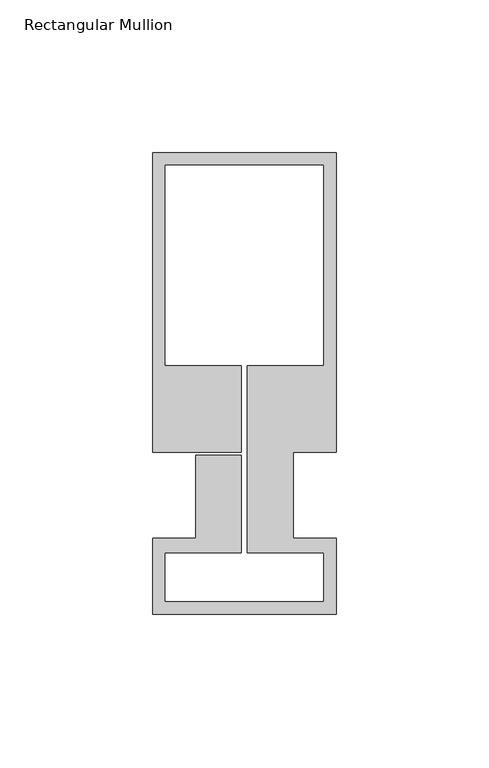
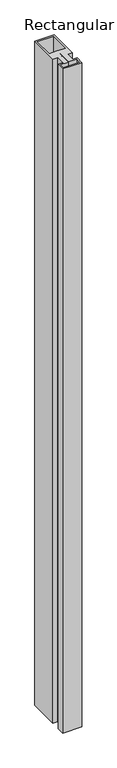
"""IFC4 building model written with IfcOpenShell, lengths in millimetres: member geometry, Rectangular Mullion : Schueco_FWS-60-HI_Mull_CovCap-20mm_Mull-85mm."""

import ifcopenshell
import ifcopenshell.guid

model = None  # the IFC model being written
_history = None  # IfcOwnerHistory: only IFC2X3 demands one
_inside = {}  # id of a spatial element -> (the spatial element, [elements in it])
_under = {}  # id of a project, library or spatial element -> (it, [spatial elements below it])
_declared = {}  # id of a project -> (the project, [libraries it declares])
_typed = {}  # id of a type object -> (the type object, [elements of that type])
_made_of = {}  # id of a material, layer set ... -> (it, [elements and type objects made of it])


def new_model(schema):
    """Start an empty IFC model of exactly this schema.

    Asked for "IFC4X3", IfcOpenShell would pick the latest addendum, in which some entities
    have other attributes; the version numbers below select the first issue.
    IFC2X3 requires an IfcOwnerHistory on every rooted entity: one is made here for all.
    """
    global model, _history
    if schema == "IFC4X3":
        model = ifcopenshell.file(schema_version=(4, 3, 0, 0))
    else:
        model = ifcopenshell.file(schema=schema)
    _inside.clear()
    _under.clear()
    _declared.clear()
    _typed.clear()
    _made_of.clear()
    _history = None
    if model.schema == "IFC2X3":
        org = make("IfcOrganization", Name="unknown")
        user = make(
            "IfcPersonAndOrganization",
            ThePerson=make("IfcPerson", FamilyName="unknown"),
            TheOrganization=org,
        )
        app = make(
            "IfcApplication",
            ApplicationDeveloper=org,
            Version="unknown",
            ApplicationFullName="unknown",
            ApplicationIdentifier="unknown",
        )
        _history = make(
            "IfcOwnerHistory",
            OwningUser=user,
            OwningApplication=app,
            ChangeAction="ADDED",
            CreationDate=0,
        )
    return model


def make(cls, **values):
    """One entity of the class cls with the attributes given. An attribute that is None is left unset."""
    return model.create_entity(
        cls, **{name: value for name, value in values.items() if value is not None}
    )


def rooted(cls, **values):
    """An entity with a GlobalId (a new one), such as an element, a storey or a relation."""
    return make(cls, GlobalId=ifcopenshell.guid.new(), OwnerHistory=_history, **values)


def si_unit(unit_type, name, prefix=None):
    """IfcSIUnit, for example si_unit("LENGTHUNIT", "METRE", prefix="MILLI")."""
    return make("IfcSIUnit", UnitType=unit_type, Prefix=prefix, Name=name)


def assignment(units):
    """IfcUnitAssignment: the units of a project."""
    return None if units is None else make("IfcUnitAssignment", Units=units)


def point(xyz):
    """IfcCartesianPoint."""
    return None if xyz is None else make("IfcCartesianPoint", Coordinates=xyz)


def direction(xyz):
    """IfcDirection."""
    return None if xyz is None else make("IfcDirection", DirectionRatios=xyz)


def frame(location, z_axis=None, x_axis=None):
    """IfcAxis2Placement3D, a coordinate frame: its origin and axes. An axis left out is left unset."""
    return make(
        "IfcAxis2Placement3D",
        Location=point(location),
        Axis=direction(z_axis),
        RefDirection=direction(x_axis),
    )


def origin():
    """The frame at (0, 0, 0) with its axes left unset."""
    return frame((0.0, 0.0, 0.0))


def place(relative_to, where):
    """IfcLocalPlacement: puts the frame where relative to a parent placement (None: the world)."""
    return make(
        "IfcLocalPlacement", PlacementRelTo=relative_to, RelativePlacement=where
    )


def context(
    kind, dimensions, precision=None, world=None, true_north=None, identifier=None
):
    """IfcGeometricRepresentationContext, for example the 3D "Model" context."""
    return make(
        "IfcGeometricRepresentationContext",
        ContextIdentifier=identifier,
        ContextType=kind,
        CoordinateSpaceDimension=dimensions,
        Precision=precision,
        WorldCoordinateSystem=world,
        TrueNorth=true_north,
    )


def project(units=None, contexts=None):
    """IfcProject with its units and contexts."""
    return rooted(
        "IfcProject",
        Name="project",
        RepresentationContexts=contexts,
        UnitsInContext=assignment(units),
    )


def spatial(cls, under=None, at=None, **own):
    """A site, building, storey or space (cls), placed at a placement, below another one or the project."""
    s = rooted(cls, ObjectPlacement=at, **own)
    if under is not None:
        _under.setdefault(under.id(), (under, []))[1].append(s)
    return s


def polyline(points):
    """IfcPolyline through the points."""
    return make("IfcPolyline", Points=[point(p) for p in points])


def outline(outer, holes=None, kind="AREA"):
    """IfcArbitraryClosedProfileDef: a profile drawn as a closed curve; with holes, ...WithVoids."""
    if holes is None:
        return make("IfcArbitraryClosedProfileDef", ProfileType=kind, OuterCurve=outer)
    return make(
        "IfcArbitraryProfileDefWithVoids",
        ProfileType=kind,
        OuterCurve=outer,
        InnerCurves=holes,
    )


def extrude(swept, where, along, depth):
    """IfcExtrudedAreaSolid: the profile swept, set in the frame where, extruded along a direction by depth."""
    return make(
        "IfcExtrudedAreaSolid",
        SweptArea=swept,
        Position=where,
        ExtrudedDirection=direction(along),
        Depth=depth,
    )


def shape(context_of_items, identifier, shape_type, items):
    """IfcShapeRepresentation: the items that make up one representation, for example the "Body"."""
    return make(
        "IfcShapeRepresentation",
        ContextOfItems=context_of_items,
        RepresentationIdentifier=identifier,
        RepresentationType=shape_type,
        Items=items,
    )


def source(mapping_origin, context_of_items, identifier, shape_type, items):
    """IfcRepresentationMap: a shape defined once, which mapped items show again and again."""
    return make(
        "IfcRepresentationMap",
        MappingOrigin=mapping_origin,
        MappedRepresentation=shape(context_of_items, identifier, shape_type, items),
    )


def transform(
    local_origin,
    x_axis=None,
    y_axis=None,
    z_axis=None,
    scale=None,
    scale2=None,
    scale3=None,
    uniform=True,
):
    """IfcCartesianTransformationOperator3D, or its non-uniform kind. x_axis, y_axis, z_axis: its Axis1, 2, 3."""
    if uniform:
        return make(
            "IfcCartesianTransformationOperator3D",
            Axis1=direction(x_axis),
            Axis2=direction(y_axis),
            LocalOrigin=point(local_origin),
            Scale=scale,
            Axis3=direction(z_axis),
        )
    return make(
        "IfcCartesianTransformationOperator3DnonUniform",
        Axis1=direction(x_axis),
        Axis2=direction(y_axis),
        LocalOrigin=point(local_origin),
        Scale=scale,
        Axis3=direction(z_axis),
        Scale2=scale2,
        Scale3=scale3,
    )


def mapped(mapping_source, mapping_target):
    """IfcMappedItem: shows the shape of a source again, moved by a transform."""
    return make(
        "IfcMappedItem", MappingSource=mapping_source, MappingTarget=mapping_target
    )


def made_of(thing, what):
    """Note that an element or type object is made of a material, layer set ...; save() writes the relation."""
    if what is not None:
        _made_of.setdefault(what.id(), (what, []))[1].append(thing)
    return thing


def element(
    cls,
    number,
    at=None,
    inside=None,
    cuts=None,
    type_object=None,
    material=None,
    context=None,
    identifier="Body",
    shape_type=None,
    held_by="IfcProductDefinitionShape",
    body=None,
    shapes=None,
    **own,
):
    """One element of the class cls, such as IfcWall. Its Tag is "e" and its number.

    at: its placement. inside: the storey or other place that contains it. cuts: it is an
    opening in that element (IfcRelVoidsElement). A single representation is given by context,
    identifier, shape_type and body (its items); several are given by shapes. held_by: the class
    of the entity that holds the representations. save() writes the other relations.
    """
    e = rooted(cls, Tag="e%d" % number, ObjectPlacement=at, **own)
    if body is not None:
        shapes = [shape(context, identifier, shape_type, body)]
    if shapes is not None:
        e.Representation = make(held_by, Representations=shapes)
    if inside is not None:
        _inside.setdefault(inside.id(), (inside, []))[1].append(e)
    if cuts is not None:
        rooted(
            "IfcRelVoidsElement", RelatingBuildingElement=cuts, RelatedOpeningElement=e
        )
    if type_object is not None:
        _typed.setdefault(type_object.id(), (type_object, []))[1].append(e)
    return made_of(e, material)


def aggregate(whole, parts):
    """IfcRelAggregates: a whole, such as a stair, and the parts it consists of."""
    return rooted("IfcRelAggregates", RelatingObject=whole, RelatedObjects=parts)


def save(model, path):
    """Write the relations noted so far, then the file.

    IfcRelAggregates (storeys below a building ...), IfcRelContainedInSpatialStructure (elements
    in a storey), IfcRelDefinesByType, IfcRelAssociatesMaterial and IfcRelDeclares: one each for
    every whole, place, type object, material and project.
    """
    for whole, parts in _under.values():
        aggregate(whole, parts)
    for where, things in _inside.values():
        rooted(
            "IfcRelContainedInSpatialStructure",
            RelatedElements=things,
            RelatingStructure=where,
        )
    for kind, things in _typed.values():
        rooted("IfcRelDefinesByType", RelatedObjects=things, RelatingType=kind)
    for what, things in _made_of.values():
        rooted("IfcRelAssociatesMaterial", RelatedObjects=things, RelatingMaterial=what)
    for by, libraries in _declared.values():
        rooted("IfcRelDeclares", RelatingContext=by, RelatedDefinitions=libraries)
    model.write(path)


def rectangular_mullion_c35b1248(model_context):
    return source(origin(), model_context, "Body", "SweptSolid", [
        extrude(outline(polyline([(0.0, 126.0), (0.0, 28.0), (-14.0, 28.0), (-14.0, -0.1), (0.0, -0.1), (0.0, -25.0), (-60.0, -25.0), (-60.0, -0.1), (-46.0, -0.1), (-46.0, 27.0), (-31.0, 27.0), (-31.0, -5.0), (-56.0, -5.0), (-56.0, -21.0), (-4.0, -21.0), (-4.0, -5.0), (-29.0, -5.0), (-29.0, 56.3), (-4.0, 56.3), (-4.0, 122.0), (-56.0, 122.0), (-56.0, 56.3), (-31.0, 56.3), (-31.0, 28.0), (-60.0, 28.0), (-60.0, 126.0), (0.0, 126.0)])), frame((0.0, 0.0, -2200.0), z_axis=(0.0, 0.0, 1.0), x_axis=(1.0, 0.0, 0.0)), (0.0, 0.0, 1.0), 2200.0),
    ])


if __name__ == "__main__":
    model = new_model("IFC4")
    model_context = context("Model", 3, world=origin())
    ifc_project = project(units=[si_unit("LENGTHUNIT", "METRE", prefix="MILLI")], contexts=[model_context])
    site = spatial("IfcSite", under=ifc_project)
    building = spatial("IfcBuilding", under=site)
    placement = place(None, origin())
    rectangular_mullion_shape = rectangular_mullion_c35b1248(model_context)
    element("IfcMember", 1, ObjectType="Rectangular Mullion : Schueco_FWS-60-HI_Mull_CovCap-20mm_Mull-85mm", at=placement, inside=building, context=model_context, shape_type="MappedRepresentation", body=[
        mapped(rectangular_mullion_shape, transform((0.0, 0.0, 0.0), x_axis=(1.0, 0.0, 0.0), y_axis=(0.0, 1.0, 0.0), z_axis=(0.0, 0.0, 1.0))),
    ])
    save(model, "model.ifc")

# Revit data of these elements
# Type "Rectangular Mullion : Schueco_FWS-60-HI_Mull_CovCap-20mm_Mull-85mm"
#   Model = "FWS 60.HI"
#   Manufacturer = "Schueco International KG"
#   Type Comments = "Mullion"
#   Schueco thermal insulation standard = "Highly thermally insulated"
#   Burglar resistance = "RC 3"
#   Thermal insulation = "to 0.90 W/(m²K)"
#   built-in parameter 1007322 = 0.495407 (stored number, unit not read)
#   built-in parameter 1007321 = 0.0524934 (stored number, unit not read)
#   built-in parameter 1007320 = 0.0524934 (stored number, unit not read)
# Element 1 (IfcMember, "Rectangular Mullion : Schueco_FWS-60-HI_Mull_CovCap-20mm_Mull-85mm")
#   Materials on its faces: "Alu"
# Materials
#   "Alu": class "Glas", colour RGB 140 140 140, transparency 0
